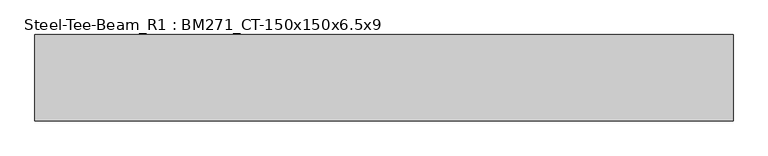
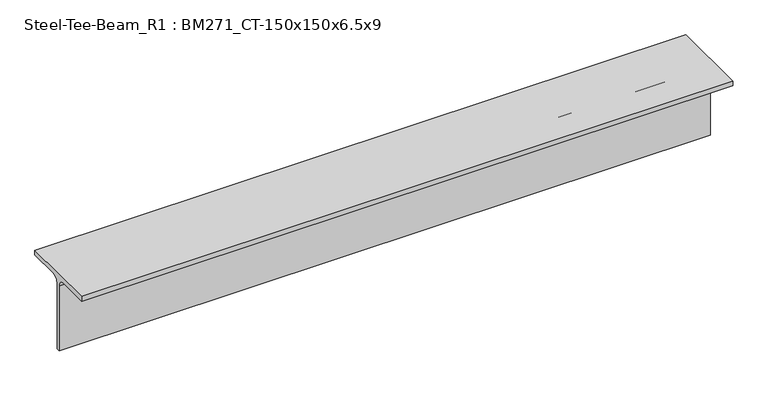
"""IFC4 building model written with IfcOpenShell, lengths in millimetres: member geometry, Steel-Tee-Beam_R1 : BM271_CT-150x150x6.5x9."""

from ifc_helpers import new_model, si_unit, point, frame, frame_2d, origin, place, context, project, spatial, polyline, circle_curve, trimmed, segment, composite_curve, outline, extrude, source, transform, mapped, element, save


def steel_tee_beam_r1_bm271_ct_150x150x6_5x9_65665e3b(model_context):
    return source(origin(), model_context, "Body", "SweptSolid", [
        extrude(outline(composite_curve([segment(polyline([(-75.0, 75.0), (75.0, 75.0), (75.0, 66.0), (16.25, 66.0)]), True, "CONTINUOUS"), segment(trimmed(circle_curve(frame_2d((16.25, 53.0)), 13.0), [point((16.25, 66.0))], [point((3.25, 53.0))], True, "CARTESIAN"), True, "CONTINUOUS"), segment(polyline([(3.25, 53.0), (3.25, -75.0), (-3.25, -75.0), (-3.25, 53.0)]), True, "CONTINUOUS"), segment(trimmed(circle_curve(frame_2d((-16.25, 53.0)), 13.0), [point((-3.25, 53.0))], [point((-16.25, 66.0))], True, "CARTESIAN"), True, "CONTINUOUS"), segment(polyline([(-16.25, 66.0), (-75.0, 66.0), (-75.0, 75.0)]), True, "CONTINUOUS")], self_intersect=False)), frame((-600.5941598, 0.0, 0.0), z_axis=(1.0, 0.0, 0.0), x_axis=(0.0, 1.0, 0.0)), (0.0, 0.0, 1.0), 1210.2197165),
    ])


if __name__ == "__main__":
    model = new_model("IFC4")
    model_context = context("Model", 3, world=origin())
    ifc_project = project(units=[si_unit("LENGTHUNIT", "METRE", prefix="MILLI")], contexts=[model_context])
    site = spatial("IfcSite", under=ifc_project)
    building = spatial("IfcBuilding", under=site)
    placement = place(None, origin())
    steel_tee_beam_r1_bm271_ct_150x150x6_5x9_shape = steel_tee_beam_r1_bm271_ct_150x150x6_5x9_65665e3b(model_context)
    element("IfcMember", 1, ObjectType="Steel-Tee-Beam_R1 : BM271_CT-150x150x6.5x9", at=placement, inside=building, context=model_context, shape_type="MappedRepresentation", body=[
        mapped(steel_tee_beam_r1_bm271_ct_150x150x6_5x9_shape, transform((0.0, 0.0, 0.0), x_axis=(1.0, 0.0, 0.0), y_axis=(0.0, 1.0, 0.0), z_axis=(0.0, 0.0, 1.0))),
    ])
    save(model, "model.ifc")

# Revit data of these elements
# Type "Steel-Tee-Beam_R1 : BM271_CT-150x150x6.5x9"
#   Keynote = "CT-150x150x6.5x9"
#   Surface Area = 0.588841 m²/m
#   Section Area = 23.3904 cm²
#   Mass per Unit Length = 18.3614 kg/m
#   Length [instance default] = 1.5240 m
#   bf = 0.1500 m
#   d = 0.1500 m
#   k = 0.0220 m
#   r = 0.0130 m
#   tf = 0.0090 m
#   tw = 0.0065 m
#   hec_material4 [instance default] = none
#   hec_material3 [instance default] = none
#   hec_material2 [instance default] = none
#   hec_material1 [instance default] = none
#   Structural Material [instance default] = Steel, 45-345
#   Assembly Code = ""
# Element 1 (IfcMember, "Steel-Tee-Beam_R1 : BM271_CT-150x150x6.5x9")
#   Structural Material = none
# Materials
#   "Steel, 45-345": class "Metal", colour RGB 189 187 185, transparency 0, Description = "Steel 345 MPa", Cost = 0
